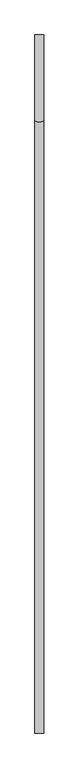
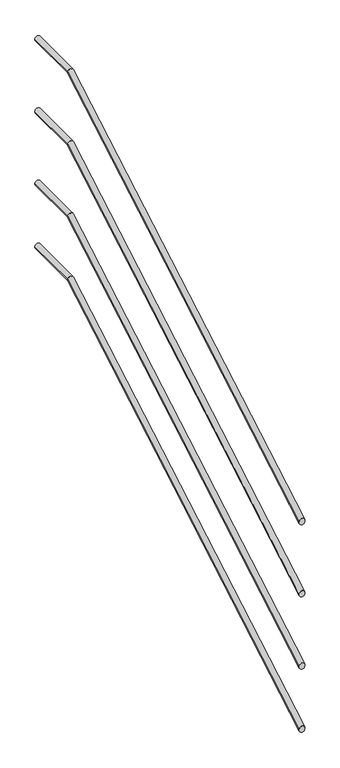
"""IFC4 building model written with IfcOpenShell, lengths in millimetres: railing geometry."""

from ifc_helpers import new_model, si_unit, frame, origin, place, context, project, spatial, circle_curve, ellipse_curve, source, transform, mapped, element, save
from ifc_brep_helpers import plane_surface, cylinder_surface, advanced_brep


def railing_e49ed630(model_context):
    return source(origin(), model_context, "Body", "AdvancedBrep", [
        advanced_brep(
        [(-1890.4, 13399.5208589, 1336.7361432), (-1860.4, 13399.5208589, 1336.7361432), (-1890.4, 15503.5584173, 2557.9030398), (-1860.4, 15503.5584173, 2557.9030398), (-1890.4, 15799.5208589, 2557.9030398), (-1860.4, 15799.5208589, 2557.9030398)],
        [
            (0, 1, ellipse_curve(frame((-1875.4, 13399.5208589, 1336.7361432), z_axis=(0.0, -1.0, 0.0), x_axis=(0.0, 0.0, -1.0)), 17.3433672, 15.0)),
            (1, 0, ellipse_curve(frame((-1875.4, 13399.5208589, 1336.7361432), z_axis=(0.0, -1.0, 0.0), x_axis=(0.0, 0.0, -1.0)), 17.3433672, 15.0)),
            (0, 2),
            (2, 3, ellipse_curve(frame((-1875.4, 15503.5584173, 2557.9030398), z_axis=(0.0, -0.9656303515230846, -0.25991926480621624), x_axis=(0.0, 0.2599192648062163, -0.9656303515230846)), 15.5338945, 15.0)),
            (3, 1),
            (3, 2, ellipse_curve(frame((-1875.4, 15503.5584173, 2557.9030398), z_axis=(0.0, -0.9656303515230846, -0.25991926480621624), x_axis=(0.0, 0.2599192648062163, -0.9656303515230846)), 15.5338945, 15.0)),
            (4, 5, circle_curve(frame((-1875.4, 15799.5208589, 2557.9030398), z_axis=(0.0, 1.0, 0.0), x_axis=(1.0, 0.0, 0.0)), 15.0)),
            (5, 4, circle_curve(frame((-1875.4, 15799.5208589, 2557.9030398), z_axis=(0.0, 1.0, 0.0), x_axis=(1.0, 0.0, 0.0)), 15.0)),
            (2, 4),
            (5, 3),
        ],
        [
            plane_surface(frame((-1875.4, 13399.5208589, 1354.0795104), z_axis=(0.0, -1.0, 0.0), x_axis=(0.0, 0.0, 1.0))),
            cylinder_surface(frame((-1875.4, 13407.0504368, 1341.1062512), z_axis=(0.0, -0.864883951565192, -0.5019718620848966), x_axis=(1.0, 0.0, 0.0)), 15.0),
            plane_surface(frame((-1875.4, 15799.5208589, 2572.9030398), z_axis=(0.0, 1.0, 0.0), x_axis=(0.0, 0.0, 1.0))),
            cylinder_surface(frame((-1875.4, 15499.5208589, 2557.9030398), z_axis=(0.0, -1.0, 0.0), x_axis=(1.0, 0.0, 0.0)), 15.0),
        ],
        [
            (0, [[1, 2]]),
            (1, [[-1, 3, 4, 5]]),
            (1, [[-2, -5, 6, -3]]),
            (2, [[7, 8]]),
            (3, [[-4, 9, -8, 10]]),
            (3, [[-6, -10, -7, -9]]),
        ],
    ),
        advanced_brep(
        [(-1890.4, 13399.5208589, 536.7361432), (-1860.4, 13399.5208589, 536.7361432), (-1890.4, 15503.5584173, 1757.9030398), (-1860.4, 15503.5584173, 1757.9030398), (-1890.4, 15799.5208589, 1757.9030398), (-1860.4, 15799.5208589, 1757.9030398)],
        [
            (0, 1, ellipse_curve(frame((-1875.4, 13399.5208589, 536.7361432), z_axis=(0.0, -1.0, 0.0), x_axis=(0.0, 0.0, -1.0)), 17.3433672, 15.0)),
            (1, 0, ellipse_curve(frame((-1875.4, 13399.5208589, 536.7361432), z_axis=(0.0, -1.0, 0.0), x_axis=(0.0, 0.0, -1.0)), 17.3433672, 15.0)),
            (0, 2),
            (2, 3, ellipse_curve(frame((-1875.4, 15503.5584173, 1757.9030398), z_axis=(0.0, -0.9656303515230846, -0.25991926480621624), x_axis=(0.0, 0.2599192648062163, -0.9656303515230846)), 15.5338945, 15.0)),
            (3, 1),
            (3, 2, ellipse_curve(frame((-1875.4, 15503.5584173, 1757.9030398), z_axis=(0.0, -0.9656303515230846, -0.25991926480621624), x_axis=(0.0, 0.2599192648062163, -0.9656303515230846)), 15.5338945, 15.0)),
            (4, 5, circle_curve(frame((-1875.4, 15799.5208589, 1757.9030398), z_axis=(0.0, 1.0, 0.0), x_axis=(1.0, 0.0, 0.0)), 15.0)),
            (5, 4, circle_curve(frame((-1875.4, 15799.5208589, 1757.9030398), z_axis=(0.0, 1.0, 0.0), x_axis=(1.0, 0.0, 0.0)), 15.0)),
            (2, 4),
            (5, 3),
        ],
        [
            plane_surface(frame((-1875.4, 13399.5208589, 554.0795104), z_axis=(0.0, -1.0, 0.0), x_axis=(0.0, 0.0, 1.0))),
            cylinder_surface(frame((-1875.4, 13407.0504368, 541.1062512), z_axis=(0.0, -0.864883951565192, -0.5019718620848966), x_axis=(1.0, 0.0, 0.0)), 15.0),
            plane_surface(frame((-1875.4, 15799.5208589, 1772.9030398), z_axis=(0.0, 1.0, 0.0), x_axis=(0.0, 0.0, 1.0))),
            cylinder_surface(frame((-1875.4, 15499.5208589, 1757.9030398), z_axis=(0.0, -1.0, 0.0), x_axis=(1.0, 0.0, 0.0)), 15.0),
        ],
        [
            (0, [[1, 2]]),
            (1, [[-1, 3, 4, 5]]),
            (1, [[-2, -5, 6, -3]]),
            (2, [[7, 8]]),
            (3, [[-4, 9, -8, 10]]),
            (3, [[-6, -10, -7, -9]]),
        ],
    ),
        advanced_brep(
        [(-1890.4, 13399.5208589, 936.7361432), (-1860.4, 13399.5208589, 936.7361432), (-1890.4, 15503.5584173, 2157.9030398), (-1860.4, 15503.5584173, 2157.9030398), (-1890.4, 15799.5208589, 2157.9030398), (-1860.4, 15799.5208589, 2157.9030398)],
        [
            (0, 1, ellipse_curve(frame((-1875.4, 13399.5208589, 936.7361432), z_axis=(0.0, -1.0, 0.0), x_axis=(0.0, 0.0, -1.0)), 17.3433672, 15.0)),
            (1, 0, ellipse_curve(frame((-1875.4, 13399.5208589, 936.7361432), z_axis=(0.0, -1.0, 0.0), x_axis=(0.0, 0.0, -1.0)), 17.3433672, 15.0)),
            (0, 2),
            (2, 3, ellipse_curve(frame((-1875.4, 15503.5584173, 2157.9030398), z_axis=(0.0, -0.9656303515230846, -0.25991926480621624), x_axis=(0.0, 0.2599192648062163, -0.9656303515230846)), 15.5338945, 15.0)),
            (3, 1),
            (3, 2, ellipse_curve(frame((-1875.4, 15503.5584173, 2157.9030398), z_axis=(0.0, -0.9656303515230846, -0.25991926480621624), x_axis=(0.0, 0.2599192648062163, -0.9656303515230846)), 15.5338945, 15.0)),
            (4, 5, circle_curve(frame((-1875.4, 15799.5208589, 2157.9030398), z_axis=(0.0, 1.0, 0.0), x_axis=(1.0, 0.0, 0.0)), 15.0)),
            (5, 4, circle_curve(frame((-1875.4, 15799.5208589, 2157.9030398), z_axis=(0.0, 1.0, 0.0), x_axis=(1.0, 0.0, 0.0)), 15.0)),
            (2, 4),
            (5, 3),
        ],
        [
            plane_surface(frame((-1875.4, 13399.5208589, 954.0795104), z_axis=(0.0, -1.0, 0.0), x_axis=(0.0, 0.0, 1.0))),
            cylinder_surface(frame((-1875.4, 13407.0504368, 941.1062512), z_axis=(0.0, -0.864883951565192, -0.5019718620848966), x_axis=(1.0, 0.0, 0.0)), 15.0),
            plane_surface(frame((-1875.4, 15799.5208589, 2172.9030398), z_axis=(0.0, 1.0, 0.0), x_axis=(0.0, 0.0, 1.0))),
            cylinder_surface(frame((-1875.4, 15499.5208589, 2157.9030398), z_axis=(0.0, -1.0, 0.0), x_axis=(1.0, 0.0, 0.0)), 15.0),
        ],
        [
            (0, [[1, 2]]),
            (1, [[-1, 3, 4, 5]]),
            (1, [[-2, -5, 6, -3]]),
            (2, [[7, 8]]),
            (3, [[-4, 9, -8, 10]]),
            (3, [[-6, -10, -7, -9]]),
        ],
    ),
        advanced_brep(
        [(-1890.4, 13399.5208589, 186.7361432), (-1860.4, 13399.5208589, 186.7361432), (-1890.4, 15503.5584173, 1407.9030398), (-1860.4, 15503.5584173, 1407.9030398), (-1890.4, 15799.5208589, 1407.9030398), (-1860.4, 15799.5208589, 1407.9030398)],
        [
            (0, 1, ellipse_curve(frame((-1875.4, 13399.5208589, 186.7361432), z_axis=(0.0, -1.0, 0.0), x_axis=(0.0, 0.0, -1.0)), 17.3433672, 15.0)),
            (1, 0, ellipse_curve(frame((-1875.4, 13399.5208589, 186.7361432), z_axis=(0.0, -1.0, 0.0), x_axis=(0.0, 0.0, -1.0)), 17.3433672, 15.0)),
            (0, 2),
            (2, 3, ellipse_curve(frame((-1875.4, 15503.5584173, 1407.9030398), z_axis=(0.0, -0.9656303515230846, -0.25991926480621624), x_axis=(0.0, 0.2599192648062163, -0.9656303515230846)), 15.5338945, 15.0)),
            (3, 1),
            (3, 2, ellipse_curve(frame((-1875.4, 15503.5584173, 1407.9030398), z_axis=(0.0, -0.9656303515230846, -0.25991926480621624), x_axis=(0.0, 0.2599192648062163, -0.9656303515230846)), 15.5338945, 15.0)),
            (4, 5, circle_curve(frame((-1875.4, 15799.5208589, 1407.9030398), z_axis=(0.0, 1.0, 0.0), x_axis=(1.0, 0.0, 0.0)), 15.0)),
            (5, 4, circle_curve(frame((-1875.4, 15799.5208589, 1407.9030398), z_axis=(0.0, 1.0, 0.0), x_axis=(1.0, 0.0, 0.0)), 15.0)),
            (2, 4),
            (5, 3),
        ],
        [
            plane_surface(frame((-1875.4, 13399.5208589, 204.0795104), z_axis=(0.0, -1.0, 0.0), x_axis=(0.0, 0.0, 1.0))),
            cylinder_surface(frame((-1875.4, 13407.0504368, 191.1062512), z_axis=(0.0, -0.864883951565192, -0.5019718620848966), x_axis=(1.0, 0.0, 0.0)), 15.0),
            plane_surface(frame((-1875.4, 15799.5208589, 1422.9030398), z_axis=(0.0, 1.0, 0.0), x_axis=(0.0, 0.0, 1.0))),
            cylinder_surface(frame((-1875.4, 15499.5208589, 1407.9030398), z_axis=(0.0, -1.0, 0.0), x_axis=(1.0, 0.0, 0.0)), 15.0),
        ],
        [
            (0, [[1, 2]]),
            (1, [[-1, 3, 4, 5]]),
            (1, [[-2, -5, 6, -3]]),
            (2, [[7, 8]]),
            (3, [[-4, 9, -8, 10]]),
            (3, [[-6, -10, -7, -9]]),
        ],
    ),
    ])


if __name__ == "__main__":
    model = new_model("IFC4")
    model_context = context("Model", 3, world=origin())
    ifc_project = project(units=[si_unit("LENGTHUNIT", "METRE", prefix="MILLI")], contexts=[model_context])
    site = spatial("IfcSite", under=ifc_project)
    building = spatial("IfcBuilding", under=site)
    placement = place(None, origin())
    railing_shape = railing_e49ed630(model_context)
    element("IfcRailing", 1, at=placement, inside=building, context=model_context, shape_type="MappedRepresentation", body=[
        mapped(railing_shape, transform((0.0, 0.0, 0.0), x_axis=(1.0, 0.0, 0.0), y_axis=(0.0, 1.0, 0.0), z_axis=(0.0, 0.0, 1.0))),
    ])
    save(model, "model.ifc")
